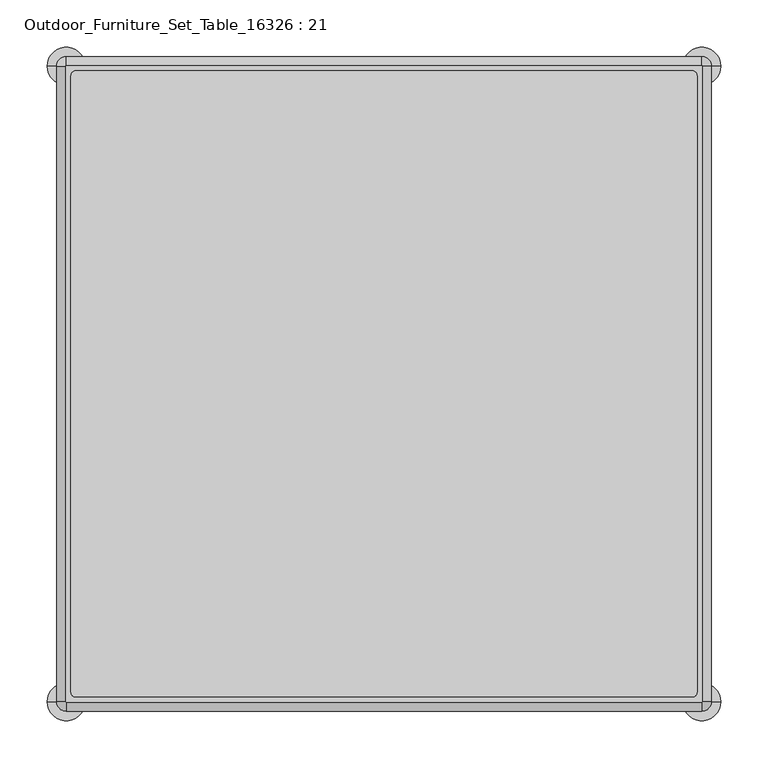
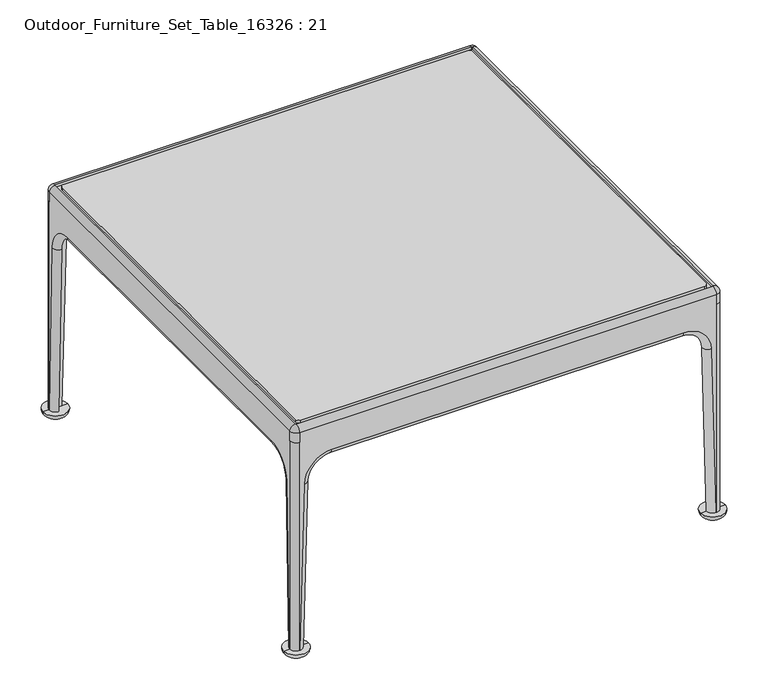
"""IFC4 building model written with IfcOpenShell, lengths in millimetres: furniture geometry, Outdoor_Furniture_Set_Table_16326 : 21."""

from ifc_helpers import new_model, si_unit, point, frame, frame_2d, origin, place, context, project, spatial, polyline, circle_curve, ellipse_curve, trimmed, segment, composite_curve, outline, extrude, source, transform, mapped, element, save
from ifc_brep_helpers import plane_surface, cylinder_surface, revolved_surface, advanced_brep


def outdoor_furniture_set_table_16326_21_ce4fcd7d(model_context):
    return source(origin(), model_context, "Body", "SolidModel", [
        extrude(outline(polyline([(337.0, 337.0), (337.0, -337.0), (-337.0, -337.0), (-337.0, 337.0), (337.0, 337.0)])), frame((0.0, 0.0, 365.0), z_axis=(0.0, 0.0, 1.0), x_axis=(1.0, 0.0, 0.0)), (0.0, 0.0, 1.0), 20.0),
        advanced_brep(
        [(-336.0, 346.0, 10.0), (-326.0034268, 336.0, 9.7382305), (-336.0, 336.0, 10.0), (-328.6370959, 346.0, 291.1779627), (-318.6405227, 336.0, 290.9161932), (-283.6525163, 336.0, 325.0), (283.6525163, 336.0, 325.0), (318.6405227, 336.0, 290.9161932), (326.0034268, 336.0, 9.7382305), (336.0, 336.0, 10.0), (336.0, 336.0, 365.0), (-336.0, 336.0, 365.0), (-283.6525163, 346.0, 335.0), (283.6525163, 346.0, 335.0), (328.6370959, 346.0, 291.1779627), (336.0, 346.0, 10.0), (-336.0, 346.0, 365.0), (-336.0, 346.0, 381.0), (336.0, 346.0, 381.0), (336.0, 346.0, 365.0), (-337.0, -336.0, 365.0), (-336.0, -337.0, 365.0), (336.0, -337.0, 365.0), (337.0, -336.0, 365.0), (337.0, 336.0, 365.0), (336.0, 337.0, 365.0), (-336.0, 337.0, 365.0), (-337.0, 336.0, 365.0), (336.0, -336.0, 365.0), (-336.0, -336.0, 365.0), (-336.0, -346.0, 381.0), (-346.0, -336.0, 381.0), (-346.0, -336.0, 365.0), (-336.0, -346.0, 365.0), (-336.0, -337.0, 390.0), (-337.0, -336.0, 390.0), (-336.0, -346.0, 10.0), (-328.6370853, -346.0, 291.1783664), (-283.6525163, -346.0, 335.0), (283.6525163, -346.0, 335.0), (328.6370853, -346.0, 291.1783664), (336.0, -346.0, 10.0), (336.0, -346.0, 365.0), (336.0, -346.0, 381.0), (336.0, -337.0, 390.0), (346.0, -336.0, 365.0), (346.0, -336.0, 381.0), (337.0, -336.0, 390.0), (346.0, -336.0, 10.0), (346.0, -328.6370959, 291.1779627), (346.0, -283.6525163, 335.0), (346.0, 283.6525163, 335.0), (346.0, 328.6370959, 291.1779627), (346.0, 336.0, 10.0), (346.0, 336.0, 365.0), (346.0, 336.0, 381.0), (337.0, 336.0, 390.0), (336.0, 337.0, 390.0), (-336.0, 337.0, 390.0), (-346.0, 336.0, 365.0), (-346.0, 336.0, 381.0), (-337.0, 336.0, 390.0), (-346.0, 336.0, 10.0), (-346.0, 328.6370853, 291.1783665), (-346.0, 283.6529202, 335.0), (-346.0, -283.6529202, 335.0), (-346.0, -328.6370853, 291.1783665), (-346.0, -336.0, 10.0), (-336.0, -326.0034268, 9.7382305), (-336.0, -336.0, 10.0), (-336.0, -318.6405121, 290.916597), (-336.0, -283.6529202, 325.0), (-336.0, 283.6529202, 325.0), (-336.0, 318.6405121, 290.916597), (-336.0, 326.0034268, 9.7382305), (326.0034268, -336.0, 9.7382305), (336.0, -336.0, 10.0), (318.6405144, -336.0, 290.9165072), (283.6525163, -336.0, 325.0), (-283.6525163, -336.0, 325.0), (-318.6405144, -336.0, 290.9165072), (-326.0034268, -336.0, 9.7382305), (336.0, 326.0034268, 9.7382305), (336.0, 318.6405227, 290.9161932), (336.0, 283.6525163, 325.0), (336.0, -283.6525163, 325.0), (336.0, -318.6405227, 290.9161932), (336.0, -326.0034268, 9.7382305)],
        [
            (0, 1, circle_curve(frame((-336.0, 336.0, 10.0), z_axis=(-0.026176948307757304, 0.0, -0.9996573249755604), x_axis=(0.9996573249755604, 0.0, -0.026176948307757304)), 10.0)),
            (1, 2),
            (2, 0),
            (0, 3),
            (3, 4, circle_curve(frame((-328.6370959, 336.0, 291.1779627), z_axis=(-0.026176948307757304, 0.0, -0.9996573249755604), x_axis=(0.9996573249755604, 0.0, -0.026176948307757304)), 10.0)),
            (4, 1),
            (4, 5, circle_curve(frame((-283.6525163, 336.0, 290.0), z_axis=(0.0, 1.0, 0.0), x_axis=(-0.9996573249749426, 0.0, 0.026176948331344894)), 35.0)),
            (5, 6),
            (6, 7, circle_curve(frame((283.6525163, 336.0, 290.0), z_axis=(0.0, 1.0, 0.0), x_axis=(0.0, 0.0, 1.0)), 35.0)),
            (7, 8),
            (8, 9),
            (9, 10),
            (10, 11),
            (11, 2),
            (3, 12, circle_curve(frame((-283.6525163, 346.0, 290.0), z_axis=(0.0, 1.0, 0.0), x_axis=(-0.9996573249749426, 0.0, 0.026176948331344894)), 45.0)),
            (12, 5, circle_curve(frame((-283.6525163, 336.0, 335.0), z_axis=(-1.0, 0.0, 0.0), x_axis=(0.0, 0.0, -1.0)), 10.0)),
            (12, 13),
            (13, 6, circle_curve(frame((283.6525163, 336.0, 335.0), z_axis=(-1.0, 0.0, 0.0), x_axis=(0.0, 0.0, -1.0)), 10.0)),
            (13, 14, circle_curve(frame((283.6525163, 346.0, 290.0), z_axis=(0.0, 1.0, 0.0), x_axis=(0.0, 0.0, 1.0)), 45.0)),
            (14, 7, circle_curve(frame((328.6370959, 336.0, 291.1779627), z_axis=(-0.02617694833120655, 0.0, 0.9996573249749463), x_axis=(-0.9996573249749463, 0.0, -0.02617694833120655)), 10.0)),
            (8, 15, circle_curve(frame((336.0, 336.0, 10.0), z_axis=(0.026176948307756947, 0.0, -0.9996573249755604), x_axis=(-0.9996573249755604, 0.0, -0.026176948307756947)), 10.0)),
            (15, 9),
            (14, 15),
            (0, 16),
            (16, 17),
            (17, 18),
            (18, 19),
            (19, 15),
            (20, 21, circle_curve(frame((-336.0, -336.0, 365.0), z_axis=(0.0, 0.0, 1.0), x_axis=(-1.0, 0.0, 0.0)), 1.0)),
            (21, 22),
            (22, 23, circle_curve(frame((336.0, -336.0, 365.0), z_axis=(0.0, 0.0, 1.0), x_axis=(0.0, -1.0, 0.0)), 1.0)),
            (23, 24),
            (24, 25, circle_curve(frame((336.0, 336.0, 365.0), z_axis=(0.0, 0.0, 1.0), x_axis=(1.0, 0.0, 0.0)), 1.0)),
            (25, 26),
            (26, 27, circle_curve(frame((-336.0, 336.0, 365.0), z_axis=(0.0, 0.0, 1.0), x_axis=(0.0, 1.0, 0.0)), 1.0)),
            (27, 20),
            (10, 28),
            (28, 29),
            (29, 11),
            (30, 31, circle_curve(frame((-336.0, -336.0, 381.0), z_axis=(0.0, 0.0, -1.0), x_axis=(-1.0, 0.0, 0.0)), 10.0)),
            (31, 32),
            (32, 33, circle_curve(frame((-336.0, -336.0, 365.0), z_axis=(0.0, 0.0, 1.0), x_axis=(-1.0, 0.0, 0.0)), 10.0)),
            (33, 30),
            (30, 34, circle_curve(frame((-336.0, -337.0, 381.0), z_axis=(-1.0, 0.0, 0.0), x_axis=(0.0, 1.0, 0.0)), 9.0)),
            (34, 35, circle_curve(frame((-336.0, -336.0, 390.0), z_axis=(0.0, 0.0, -1.0), x_axis=(-1.0, 0.0, 0.0)), 1.0)),
            (35, 31, circle_curve(frame((-337.0, -336.0, 381.0), z_axis=(0.0, -1.0, 0.0), x_axis=(1.0, 0.0, 0.0)), 9.0)),
            (33, 36),
            (36, 37),
            (37, 38, circle_curve(frame((-283.6525163, -346.0, 290.0), z_axis=(0.0, 1.0, 0.0), x_axis=(0.0, 0.0, 1.0)), 45.0)),
            (38, 39),
            (39, 40, circle_curve(frame((283.6525163, -346.0, 290.0), z_axis=(0.0, 1.0, 0.0), x_axis=(0.9996570900025821, 0.0, 0.026185920025262065)), 45.0)),
            (40, 41),
            (41, 42),
            (42, 43),
            (43, 30),
            (43, 44, circle_curve(frame((336.0, -337.0, 381.0), z_axis=(-1.0, 0.0, 0.0), x_axis=(0.0, 1.0, 0.0)), 9.0)),
            (44, 34),
            (42, 45, circle_curve(frame((336.0, -336.0, 365.0), z_axis=(0.0, 0.0, 1.0), x_axis=(0.0, -1.0, 0.0)), 10.0)),
            (45, 46),
            (46, 43, circle_curve(frame((336.0, -336.0, 381.0), z_axis=(0.0, 0.0, -1.0), x_axis=(0.0, -1.0, 0.0)), 10.0)),
            (46, 47, circle_curve(frame((337.0, -336.0, 381.0), z_axis=(0.0, -1.0, 0.0), x_axis=(-1.0, 0.0, 0.0)), 9.0)),
            (47, 44, circle_curve(frame((336.0, -336.0, 390.0), z_axis=(0.0, 0.0, -1.0), x_axis=(0.0, -1.0, 0.0)), 1.0)),
            (45, 48),
            (48, 49),
            (49, 50, circle_curve(frame((346.0, -283.6525163, 290.0), z_axis=(-1.0, 0.0, 0.0), x_axis=(0.0, 0.0, 1.0)), 45.0)),
            (50, 51),
            (51, 52, circle_curve(frame((346.0, 283.6525163, 290.0), z_axis=(-1.0, 0.0, 0.0), x_axis=(0.0, 0.9996573249749827, 0.0261769483298142)), 45.0)),
            (52, 53),
            (53, 54),
            (54, 55),
            (55, 46),
            (55, 56, circle_curve(frame((337.0, 336.0, 381.0), z_axis=(0.0, -1.0, 0.0), x_axis=(-1.0, 0.0, 0.0)), 9.0)),
            (56, 47),
            (54, 19, circle_curve(frame((336.0, 336.0, 365.0), z_axis=(0.0, 0.0, 1.0), x_axis=(1.0, 0.0, 0.0)), 10.0)),
            (18, 55, circle_curve(frame((336.0, 336.0, 381.0), z_axis=(0.0, 0.0, -1.0), x_axis=(1.0, 0.0, 0.0)), 10.0)),
            (18, 57, circle_curve(frame((336.0, 337.0, 381.0), z_axis=(1.0, 0.0, 0.0), x_axis=(0.0, -1.0, 0.0)), 9.0)),
            (57, 56, circle_curve(frame((336.0, 336.0, 390.0), z_axis=(0.0, 0.0, -1.0), x_axis=(1.0, 0.0, 0.0)), 1.0)),
            (17, 58, circle_curve(frame((-336.0, 337.0, 381.0), z_axis=(1.0, 0.0, 0.0), x_axis=(0.0, -1.0, 0.0)), 9.0)),
            (58, 57),
            (16, 59, circle_curve(frame((-336.0, 336.0, 365.0), z_axis=(0.0, 0.0, 1.0), x_axis=(0.0, 1.0, 0.0)), 10.0)),
            (59, 60),
            (60, 17, circle_curve(frame((-336.0, 336.0, 381.0), z_axis=(0.0, 0.0, -1.0), x_axis=(0.0, 1.0, 0.0)), 10.0)),
            (60, 61, circle_curve(frame((-337.0, 336.0, 381.0), z_axis=(0.0, 1.0, 0.0), x_axis=(1.0, 0.0, 0.0)), 9.0)),
            (61, 58, circle_curve(frame((-336.0, 336.0, 390.0), z_axis=(0.0, 0.0, -1.0), x_axis=(0.0, 1.0, 0.0)), 1.0)),
            (31, 60),
            (59, 62),
            (62, 63),
            (63, 64, circle_curve(frame((-346.0, 283.6529202, 290.0004146), z_axis=(1.0, 0.0, 0.0), x_axis=(0.0, 0.0, 1.0)), 44.9995854)),
            (64, 65),
            (65, 66, circle_curve(frame((-346.0, -283.6529202, 290.0004146), z_axis=(1.0, 0.0, 0.0), x_axis=(0.0, -0.9996573249744442, 0.026176948350383943)), 44.9995854)),
            (66, 67),
            (67, 32),
            (35, 61),
            (34, 21),
            (20, 35),
            (44, 22),
            (47, 23),
            (56, 24),
            (57, 25),
            (58, 26),
            (61, 27),
            (67, 68, circle_curve(frame((-336.0, -336.0, 10.0), z_axis=(0.0, -0.026176948307878527, -0.9996573249755571), x_axis=(0.0, -0.9996573249755571, 0.026176948307878527)), 10.0)),
            (68, 69),
            (69, 67),
            (66, 70, circle_curve(frame((-336.0, -328.6370853, 291.1783665), z_axis=(0.0, -0.026176948307878527, -0.9996573249755571), x_axis=(0.0, -0.9996573249755571, 0.026176948307878527)), 10.0)),
            (70, 68),
            (70, 71, circle_curve(frame((-336.0, -283.6529202, 290.0004146), z_axis=(-1.0, 0.0, 0.0), x_axis=(0.0, -0.9996573249744442, 0.026176948350383943)), 34.9995854)),
            (71, 72),
            (72, 73, circle_curve(frame((-336.0, 283.6529202, 290.0004146), z_axis=(-1.0, 0.0, 0.0), x_axis=(0.0, 0.0, 1.0)), 34.9995854)),
            (73, 74),
            (74, 2),
            (29, 69),
            (65, 71, circle_curve(frame((-336.0, -283.6529202, 335.0), z_axis=(0.0, -1.0, 0.0), x_axis=(0.0, 0.0, 1.0)), 10.0)),
            (64, 72, circle_curve(frame((-336.0, 283.6529202, 335.0), z_axis=(0.0, -1.0, 0.0), x_axis=(0.0, 0.0, 1.0)), 10.0)),
            (63, 73, circle_curve(frame((-336.0, 328.6370853, 291.1783665), z_axis=(0.0, -0.026176948350188068, 0.9996573249744493), x_axis=(0.0, 0.9996573249744493, 0.026176948350188068)), 10.0)),
            (74, 62, circle_curve(frame((-336.0, 336.0, 10.0), z_axis=(0.0, 0.026176948307879942, -0.9996573249755571), x_axis=(0.0, 0.9996573249755571, 0.026176948307879942)), 10.0)),
            (62, 2),
            (41, 75, circle_curve(frame((336.0, -336.0, 10.0), z_axis=(0.026176948314418396, 0.0, -0.999657324975386), x_axis=(-0.999657324975386, 0.0, -0.026176948314418396)), 10.0)),
            (75, 76),
            (76, 41),
            (40, 77, circle_curve(frame((328.6370853, -336.0, 291.1783664), z_axis=(0.02618592002526207, 0.0, -0.9996570900025821), x_axis=(-0.9996570900025821, 0.0, -0.02618592002526207)), 10.0)),
            (77, 75),
            (77, 78, circle_curve(frame((283.6525163, -336.0, 290.0), z_axis=(0.0, -1.0, 0.0), x_axis=(0.9996570900025821, 0.0, 0.026185920025262065)), 35.0)),
            (78, 79),
            (79, 80, circle_curve(frame((-283.6525163, -336.0, 290.0), z_axis=(0.0, -1.0, 0.0), x_axis=(0.0, 0.0, 1.0)), 35.0)),
            (80, 81),
            (81, 69),
            (28, 76),
            (39, 78, circle_curve(frame((283.6525163, -336.0, 335.0), z_axis=(1.0, 0.0, 0.0), x_axis=(0.0, 0.0, -1.0)), 10.0)),
            (38, 79, circle_curve(frame((-283.6525163, -336.0, 335.0), z_axis=(1.0, 0.0, 0.0), x_axis=(0.0, 0.0, -1.0)), 10.0)),
            (37, 80, circle_curve(frame((-328.6370853, -336.0, 291.1783664), z_axis=(0.02618592006476948, 0.0, 0.9996570900015472), x_axis=(0.9996570900015472, 0.0, -0.02618592006476948)), 10.0)),
            (81, 36, circle_curve(frame((-336.0, -336.0, 10.0), z_axis=(-0.02617694831409382, 0.0, -0.9996573249753945), x_axis=(0.9996573249753945, 0.0, -0.02617694831409382)), 10.0)),
            (36, 69),
            (53, 82, circle_curve(frame((336.0, 336.0, 10.0), z_axis=(0.0, 0.026176948307602733, -0.9996573249755644), x_axis=(0.0, -0.9996573249755644, -0.026176948307602733)), 10.0)),
            (82, 9),
            (9, 53),
            (52, 83, circle_curve(frame((336.0, 328.6370959, 291.1779627), z_axis=(0.0, 0.026176948307602733, -0.9996573249755644), x_axis=(0.0, -0.9996573249755644, -0.026176948307602733)), 10.0)),
            (83, 82),
            (83, 84, circle_curve(frame((336.0, 283.6525163, 290.0), z_axis=(1.0, 0.0, 0.0), x_axis=(0.0, 0.9996573249749827, 0.0261769483298142)), 35.0)),
            (84, 85),
            (85, 86, circle_curve(frame((336.0, -283.6525163, 290.0), z_axis=(1.0, 0.0, 0.0), x_axis=(0.0, 0.0, 1.0)), 35.0)),
            (86, 87),
            (87, 76),
            (51, 84, circle_curve(frame((336.0, 283.6525163, 335.0), z_axis=(0.0, 1.0, 0.0), x_axis=(0.0, 0.0, -1.0)), 10.0)),
            (50, 85, circle_curve(frame((336.0, -283.6525163, 335.0), z_axis=(0.0, 1.0, 0.0), x_axis=(0.0, 0.0, -1.0)), 10.0)),
            (49, 86, circle_curve(frame((336.0, -328.6370959, 291.1779627), z_axis=(0.0, 0.026176948331144378, 0.999657324974948), x_axis=(0.0, 0.999657324974948, -0.026176948331144378)), 10.0)),
            (87, 48, circle_curve(frame((336.0, -336.0, 10.0), z_axis=(0.0, -0.0261769483077446, -0.9996573249755608), x_axis=(0.0, 0.9996573249755608, -0.0261769483077446)), 10.0)),
            (48, 76),
            (15, 53, circle_curve(frame((336.0, 336.0, 10.0), z_axis=(0.0, 0.0, -1.0), x_axis=(1.0, 0.0, 0.0)), 10.0)),
            (48, 41, circle_curve(frame((336.0, -336.0, 10.0), z_axis=(0.0, 0.0, -1.0), x_axis=(1.0, 0.0, 0.0)), 10.0)),
            (36, 67, circle_curve(frame((-336.0, -336.0, 10.0), z_axis=(0.0, 0.0, -1.0), x_axis=(1.0, 0.0, 0.0)), 10.0)),
            (62, 0, circle_curve(frame((-336.0, 336.0, 10.0), z_axis=(0.0, 0.0, -1.0), x_axis=(1.0, 0.0, 0.0)), 10.0)),
        ],
        [
            plane_surface(frame((-336.0, 346.0, 10.0), z_axis=(-0.026176948307757304, 0.0, -0.9996573249755604), x_axis=(0.0, 1.0, 0.0))),
            cylinder_surface(frame((-336.0, 336.0, 10.0), z_axis=(-0.026176948307757304, 0.0, -0.9996573249755604), x_axis=(0.9996573249755604, 0.0, -0.026176948307757304)), 10.0),
            plane_surface(frame((-326.0034268, 336.0, 9.7382305), z_axis=(0.0, -1.0, 0.0), x_axis=(0.02617694830775733, 0.0, 0.9996573249755604))),
            revolved_surface(trimmed(ellipse_curve(frame((-328.6370959, 336.0, 291.1779627), z_axis=(-0.026176948331344894, 0.0, -0.9996573249749426), x_axis=(0.9996573249749426, 0.0, -0.026176948331344894)), 10.0, 10.0), [point((-328.6370959, 346.0, 291.1779627))], [point((-318.6405227, 336.0, 290.9161932))], True, "CARTESIAN"), (-283.6525163, 346.0, 290.0), (0.0, 1.0, 0.0)),
            cylinder_surface(frame((-283.6525163, 336.0, 335.0), z_axis=(-1.0, 0.0, 0.0), x_axis=(0.0, 0.0, -1.0)), 10.0),
            revolved_surface(trimmed(ellipse_curve(frame((283.6525163, 336.0, 335.0), z_axis=(-1.0, 0.0, 0.0), x_axis=(0.0, 0.0, -1.0)), 10.0, 10.0), [point((283.6525163, 346.0, 335.0))], [point((283.6525163, 336.0, 325.0))], True, "CARTESIAN"), (283.6525163, 346.0, 290.0), (0.0, 1.0, 0.0)),
            plane_surface(frame((336.0, 346.0, 10.0), z_axis=(0.026176948307756947, 0.0, -0.9996573249755604), x_axis=(0.0, 1.0, 0.0))),
            cylinder_surface(frame((328.6370959, 336.0, 291.1779627), z_axis=(-0.026176948307756947, 0.0, 0.9996573249755604), x_axis=(-0.9996573249755604, 0.0, -0.026176948307756947)), 10.0),
            plane_surface(frame((-283.6525163, 346.0, 335.0), z_axis=(0.0, 1.0, 0.0), x_axis=(-1.0, 0.0, 0.0))),
            plane_surface(frame((-336.0, 346.0, 365.0), z_axis=(0.0, 0.0, 1.0), x_axis=(0.0, -1.0, 0.0))),
            cylinder_surface(frame((-336.0, -336.0, 0.0), z_axis=(0.0, 0.0, 1.0), x_axis=(-1.0, 0.0, 0.0)), 10.0),
            revolved_surface(trimmed(ellipse_curve(frame((-337.0, -336.0, 381.0), z_axis=(0.0, 1.0, 0.0), x_axis=(1.0, 0.0, 0.0)), 9.0, 9.0), [point((-346.0, -336.0, 381.0))], [point((-337.0, -336.0, 390.0))], True, "CARTESIAN"), (-336.0, -336.0, 0.0), (0.0, 0.0, 1.0)),
            plane_surface(frame((-336.0, -346.0, 365.0), z_axis=(0.0, -1.0, 0.0), x_axis=(1.0, 0.0, 0.0))),
            cylinder_surface(frame((-336.0, -337.0, 381.0), z_axis=(-1.0, 0.0, 0.0), x_axis=(0.0, 1.0, 0.0)), 9.0),
            cylinder_surface(frame((336.0, -336.0, 0.0), z_axis=(0.0, 0.0, 1.0), x_axis=(0.0, -1.0, 0.0)), 10.0),
            revolved_surface(trimmed(ellipse_curve(frame((336.0, -337.0, 381.0), z_axis=(-1.0, 0.0, 0.0), x_axis=(0.0, 1.0, 0.0)), 9.0, 9.0), [point((336.0, -346.0, 381.0))], [point((336.0, -337.0, 390.0))], True, "CARTESIAN"), (336.0, -336.0, 0.0), (0.0, 0.0, 1.0)),
            plane_surface(frame((346.0, -336.0, 365.0), z_axis=(1.0, 0.0, 0.0), x_axis=(0.0, 1.0, 0.0))),
            cylinder_surface(frame((337.0, -336.0, 381.0), z_axis=(0.0, -1.0, 0.0), x_axis=(-1.0, 0.0, 0.0)), 9.0),
            cylinder_surface(frame((336.0, 336.0, 0.0), z_axis=(0.0, 0.0, 1.0), x_axis=(1.0, 0.0, 0.0)), 10.0),
            revolved_surface(trimmed(ellipse_curve(frame((337.0, 336.0, 381.0), z_axis=(0.0, -1.0, 0.0), x_axis=(-1.0, 0.0, 0.0)), 9.0, 9.0), [point((346.0, 336.0, 381.0))], [point((337.0, 336.0, 390.0))], True, "CARTESIAN"), (336.0, 336.0, 0.0), (0.0, 0.0, 1.0)),
            cylinder_surface(frame((336.0, 337.0, 381.0), z_axis=(1.0, 0.0, 0.0), x_axis=(0.0, -1.0, 0.0)), 9.0),
            cylinder_surface(frame((-336.0, 336.0, 0.0), z_axis=(0.0, 0.0, 1.0), x_axis=(0.0, 1.0, 0.0)), 10.0),
            revolved_surface(trimmed(ellipse_curve(frame((-336.0, 337.0, 381.0), z_axis=(1.0, 0.0, 0.0), x_axis=(0.0, -1.0, 0.0)), 9.0, 9.0), [point((-336.0, 346.0, 381.0))], [point((-336.0, 337.0, 390.0))], True, "CARTESIAN"), (-336.0, 336.0, 0.0), (0.0, 0.0, 1.0)),
            plane_surface(frame((-346.0, 336.0, 365.0), z_axis=(-1.0, 0.0, 0.0), x_axis=(0.0, -1.0, 0.0))),
            cylinder_surface(frame((-337.0, 336.0, 381.0), z_axis=(0.0, 1.0, 0.0), x_axis=(1.0, 0.0, 0.0)), 9.0),
            revolved_surface(polyline([(-337.0, -336.0, 390.0), (-337.0, -336.0, 365.0)]), (-336.0, -336.0, 0.0), (0.0, 0.0, 1.0)),
            plane_surface(frame((-336.0, -337.0, 390.0), z_axis=(0.0, 1.0, 0.0), x_axis=(1.0, 0.0, 0.0))),
            revolved_surface(polyline([(336.0, -337.0, 390.0), (336.0, -337.0, 365.0)]), (336.0, -336.0, 0.0), (0.0, 0.0, 1.0)),
            plane_surface(frame((337.0, -336.0, 390.0), z_axis=(-1.0, 0.0, 0.0), x_axis=(0.0, 1.0, 0.0))),
            revolved_surface(polyline([(337.0, 336.0, 390.0), (337.0, 336.0, 365.0)]), (336.0, 336.0, 0.0), (0.0, 0.0, 1.0)),
            plane_surface(frame((336.0, 337.0, 390.0), z_axis=(0.0, -1.0, 0.0), x_axis=(-1.0, 0.0, 0.0))),
            revolved_surface(polyline([(-336.0, 337.0, 390.0), (-336.0, 337.0, 365.0)]), (-336.0, 336.0, 0.0), (0.0, 0.0, 1.0)),
            plane_surface(frame((-337.0, 336.0, 390.0), z_axis=(1.0, 0.0, 0.0), x_axis=(0.0, -1.0, 0.0))),
            plane_surface(frame((-346.0, -336.0, 10.0), z_axis=(0.0, -0.026176948307878527, -0.9996573249755571), x_axis=(1.0, 0.0, 0.0))),
            cylinder_surface(frame((-336.0, -336.0, 10.0), z_axis=(0.0, -0.026176948307878527, -0.9996573249755571), x_axis=(0.0, -0.9996573249755571, 0.026176948307878527)), 10.0),
            plane_surface(frame((-336.0, -326.0034268, 9.7382305), z_axis=(1.0, 0.0, 0.0), x_axis=(0.0, 0.026176948307878613, 0.9996573249755571))),
            revolved_surface(trimmed(ellipse_curve(frame((-336.0, -328.6370853, 291.1783665), z_axis=(0.0, -0.026176948350383943, -0.9996573249744442), x_axis=(0.0, -0.9996573249744442, 0.026176948350383943)), 10.0, 10.0), [point((-346.0, -328.6370853, 291.1783665))], [point((-336.0, -318.6405121, 290.916597))], True, "CARTESIAN"), (-346.0, -283.6529202, 290.0004146), (-1.0, 0.0, 0.0)),
            cylinder_surface(frame((-336.0, -283.6529202, 335.0), z_axis=(0.0, -1.0, 0.0), x_axis=(0.0, 0.0, 1.0)), 10.0),
            revolved_surface(trimmed(ellipse_curve(frame((-336.0, 283.6529202, 335.0), z_axis=(0.0, -1.0, 0.0), x_axis=(0.0, 0.0, 1.0)), 10.0, 10.0), [point((-346.0, 283.6529202, 335.0))], [point((-336.0, 283.6529202, 325.0))], True, "CARTESIAN"), (-346.0, 283.6529202, 290.0004146), (-1.0, 0.0, 0.0)),
            plane_surface(frame((-346.0, 336.0, 10.0), z_axis=(0.0, 0.026176948307879942, -0.9996573249755571), x_axis=(1.0, 0.0, 0.0))),
            cylinder_surface(frame((-336.0, 328.6370853, 291.1783665), z_axis=(0.0, -0.026176948307879942, 0.9996573249755571), x_axis=(0.0, 0.9996573249755571, 0.026176948307879942)), 10.0),
            plane_surface(frame((336.0, -346.0, 10.0), z_axis=(0.026176948314418396, 0.0, -0.999657324975386), x_axis=(0.0, -1.0, 0.0))),
            cylinder_surface(frame((336.0, -336.0, 10.0), z_axis=(0.026176948314418396, 0.0, -0.999657324975386), x_axis=(-0.999657324975386, 0.0, -0.026176948314418396)), 10.0),
            plane_surface(frame((326.0034268, -336.0, 9.7382305), z_axis=(0.0, 1.0, 0.0), x_axis=(-0.02617694831441851, 0.0, 0.999657324975386))),
            revolved_surface(trimmed(ellipse_curve(frame((328.6370853, -336.0, 291.1783664), z_axis=(0.02618592002526207, 0.0, -0.9996570900025821), x_axis=(-0.9996570900025821, 0.0, -0.02618592002526207)), 10.0, 10.0), [point((328.6370853, -346.0, 291.1783664))], [point((318.6405144, -336.0, 290.9165072))], True, "CARTESIAN"), (283.6525163, -346.0, 290.0), (0.0, -1.0, 0.0)),
            cylinder_surface(frame((283.6525163, -336.0, 335.0), z_axis=(1.0, 0.0, 0.0), x_axis=(0.0, 0.0, -1.0)), 10.0),
            revolved_surface(trimmed(ellipse_curve(frame((-283.6525163, -336.0, 335.0), z_axis=(1.0, 0.0, 0.0), x_axis=(0.0, 0.0, -1.0)), 10.0, 10.0), [point((-283.6525163, -346.0, 335.0))], [point((-283.6525163, -336.0, 325.0))], True, "CARTESIAN"), (-283.6525163, -346.0, 290.0), (0.0, -1.0, 0.0)),
            plane_surface(frame((-336.0, -346.0, 10.0), z_axis=(-0.026176948314093826, 0.0, -0.9996573249753945), x_axis=(0.0, -1.0, 0.0))),
            cylinder_surface(frame((-328.6370853, -336.0, 291.1783664), z_axis=(0.02617694831409382, 0.0, 0.9996573249753945), x_axis=(0.9996573249753945, 0.0, -0.02617694831409382)), 10.0),
            plane_surface(frame((346.0, 336.0, 10.0), z_axis=(0.0, 0.026176948307602733, -0.9996573249755644), x_axis=(1.0, 0.0, 0.0))),
            cylinder_surface(frame((336.0, 336.0, 10.0), z_axis=(0.0, 0.026176948307602733, -0.9996573249755644), x_axis=(0.0, -0.9996573249755644, -0.026176948307602733)), 10.0),
            plane_surface(frame((336.0, 326.0034268, 9.7382305), z_axis=(-1.0, 0.0, 0.0), x_axis=(0.0, -0.02617694830760276, 0.9996573249755644))),
            revolved_surface(trimmed(ellipse_curve(frame((336.0, 328.6370959, 291.1779627), z_axis=(0.0, 0.0261769483298142, -0.9996573249749827), x_axis=(0.0, -0.9996573249749827, -0.0261769483298142)), 10.0, 10.0), [point((346.0, 328.6370959, 291.1779627))], [point((336.0, 318.6405227, 290.9161932))], True, "CARTESIAN"), (346.0, 283.6525163, 290.0), (1.0, 0.0, 0.0)),
            cylinder_surface(frame((336.0, 283.6525163, 335.0), z_axis=(0.0, 1.0, 0.0), x_axis=(0.0, 0.0, -1.0)), 10.0),
            revolved_surface(trimmed(ellipse_curve(frame((336.0, -283.6525163, 335.0), z_axis=(0.0, 1.0, 0.0), x_axis=(0.0, 0.0, -1.0)), 10.0, 10.0), [point((346.0, -283.6525163, 335.0))], [point((336.0, -283.6525163, 325.0))], True, "CARTESIAN"), (346.0, -283.6525163, 290.0), (1.0, 0.0, 0.0)),
            plane_surface(frame((346.0, -336.0, 10.0), z_axis=(0.0, -0.0261769483077446, -0.9996573249755608), x_axis=(1.0, 0.0, 0.0))),
            cylinder_surface(frame((336.0, -328.6370959, 291.1779627), z_axis=(0.0, 0.0261769483077446, 0.9996573249755608), x_axis=(0.0, 0.9996573249755608, -0.0261769483077446)), 10.0),
            plane_surface(frame((336.0, 336.0, 10.0), z_axis=(0.0, 0.0, -1.0), x_axis=(-1.0, 0.0, 0.0))),
            cylinder_surface(frame((336.0, 336.0, 10.0), z_axis=(0.0, 0.0, 1.0), x_axis=(1.0, 0.0, 0.0)), 10.0),
            cylinder_surface(frame((336.0, -336.0, 0.0), z_axis=(0.0, 0.0, 1.0), x_axis=(1.0, 0.0, 0.0)), 10.0),
            cylinder_surface(frame((-336.0, -336.0, 0.0), z_axis=(0.0, 0.0, 1.0), x_axis=(1.0, 0.0, 0.0)), 10.0),
            cylinder_surface(frame((-336.0, 336.0, 0.0), z_axis=(0.0, 0.0, 1.0), x_axis=(1.0, 0.0, 0.0)), 10.0),
        ],
        [
            (0, [[1, 2, 3]]),
            (1, [[-1, 4, 5, 6]]),
            (2, [[-2, -6, 7, 8, 9, 10, 11, 12, 13, 14]]),
            (3, [[-5, 15, 16, -7]]),
            (4, [[-8, -16, 17, 18]]),
            (5, [[-9, -18, 19, 20]]),
            (6, [[-11, 21, 22]]),
            (7, [[-10, -20, 23, -21]]),
            (8, [[-4, 24, 25, 26, 27, 28, -23, -19, -17, -15]]),
            (9, [[29, 30, 31, 32, 33, 34, 35, 36], [-13, 37, 38, 39]]),
            (10, [[40, 41, 42, 43]]),
            (11, [[-40, 44, 45, 46]]),
            (12, [[-43, 47, 48, 49, 50, 51, 52, 53, 54, 55]]),
            (13, [[-44, -55, 56, 57]]),
            (14, [[-54, 58, 59, 60]]),
            (15, [[-56, -60, 61, 62]]),
            (16, [[-59, 63, 64, 65, 66, 67, 68, 69, 70, 71]]),
            (17, [[-61, -71, 72, 73]]),
            (18, [[-70, 74, -27, 75]]),
            (19, [[-72, -75, 76, 77]]),
            (20, [[-76, -26, 78, 79]]),
            (21, [[-25, 80, 81, 82]]),
            (22, [[-78, -82, 83, 84]]),
            (23, [[-41, 85, -81, 86, 87, 88, 89, 90, 91, 92]]),
            (24, [[-46, 93, -83, -85]]),
            (25, [[-45, 94, -29, 95]]),
            (26, [[-57, 96, -30, -94]]),
            (27, [[-62, 97, -31, -96]]),
            (28, [[-73, 98, -32, -97]]),
            (29, [[-77, 99, -33, -98]]),
            (30, [[-79, 100, -34, -99]]),
            (31, [[-84, 101, -35, -100]]),
            (32, [[-93, -95, -36, -101]]),
            (33, [[102, 103, 104]]),
            (34, [[-102, -91, 105, 106]]),
            (35, [[-103, -106, 107, 108, 109, 110, 111, -14, -39, 112]]),
            (36, [[-105, -90, 113, -107]]),
            (37, [[-108, -113, -89, 114]]),
            (38, [[-109, -114, -88, 115]]),
            (39, [[-111, 116, 117]]),
            (40, [[-110, -115, -87, -116]]),
            (41, [[118, 119, 120]]),
            (42, [[-118, -52, 121, 122]]),
            (43, [[-119, -122, 123, 124, 125, 126, 127, -112, -38, 128]]),
            (44, [[-121, -51, 129, -123]]),
            (45, [[-124, -129, -50, 130]]),
            (46, [[-125, -130, -49, 131]]),
            (47, [[-127, 132, 133]]),
            (48, [[-126, -131, -48, -132]]),
            (49, [[134, 135, 136]]),
            (50, [[-134, -68, 137, 138]]),
            (51, [[-135, -138, 139, 140, 141, 142, 143, -128, -37, -12]]),
            (52, [[-137, -67, 144, -139]]),
            (53, [[-140, -144, -66, 145]]),
            (54, [[-141, -145, -65, 146]]),
            (55, [[-143, 147, 148]]),
            (56, [[-142, -146, -64, -147]]),
            (57, [[149, -136, -22]]),
            (57, [[150, -120, -148]]),
            (57, [[151, -104, -133]]),
            (57, [[152, -3, -117]]),
            (58, [[-149, -28, -74, -69]]),
            (59, [[-150, -63, -58, -53]]),
            (60, [[-151, -47, -42, -92]]),
            (61, [[-152, -86, -80, -24]]),
        ],
    ),
        extrude(outline(composite_curve([segment(polyline([(326.0228318, -331.0), (-326.0, -331.0)]), True, "CONTINUOUS"), segment(trimmed(circle_curve(frame_2d((-326.0, -326.0)), 5.0), [point((-326.0, -331.0))], [point((-331.0, -326.0))], False, "CARTESIAN"), True, "CONTINUOUS"), segment(polyline([(-331.0, -326.0), (-331.0, 326.0)]), True, "CONTINUOUS"), segment(trimmed(circle_curve(frame_2d((-326.0, 326.0)), 5.0), [point((-331.0, 326.0))], [point((-326.0, 331.0))], False, "CARTESIAN"), True, "CONTINUOUS"), segment(polyline([(-326.0, 331.0), (326.0228318, 331.0)]), True, "CONTINUOUS"), segment(trimmed(circle_curve(frame_2d((326.0228318, 326.0)), 5.0), [point((326.0228318, 331.0))], [point((331.0228318, 326.0))], False, "CARTESIAN"), True, "CONTINUOUS"), segment(polyline([(331.0228318, 326.0), (331.0228318, -326.0)]), True, "CONTINUOUS"), segment(trimmed(circle_curve(frame_2d((326.0228318, -326.0)), 5.0), [point((331.0228318, -326.0))], [point((326.0228318, -331.0))], False, "CARTESIAN"), True, "CONTINUOUS")], self_intersect=False)), frame((0.0, 0.0, 385.0), z_axis=(0.0, 0.0, 1.0), x_axis=(1.0, 0.0, 0.0)), (0.0, 0.0, 1.0), 5.0),
        advanced_brep(
        [(-316.0, -336.0, 10.0), (-356.0, -336.0, 10.0), (-336.0, -336.0, 10.0), (-326.0, -336.0, 0.0), (-346.0, -336.0, 0.0), (-336.0, -336.0, 0.0)],
        [
            (0, 1, circle_curve(frame((-336.0, -336.0, 10.0), z_axis=(0.0, 0.0, 1.0), x_axis=(-1.0, 0.0, 0.0)), 20.0)),
            (1, 2),
            (2, 0),
            (1, 0, circle_curve(frame((-336.0, -336.0, 10.0), z_axis=(0.0, 0.0, 1.0), x_axis=(-1.0, 0.0, 0.0)), 20.0)),
            (3, 4, circle_curve(frame((-336.0, -336.0, 0.0), z_axis=(0.0, 0.0, 1.0), x_axis=(-1.0, 0.0, 0.0)), 10.0)),
            (4, 1, circle_curve(frame((-346.0, -336.0, 10.0), z_axis=(0.0, 1.0, 0.0), x_axis=(-1.0, 0.0, 0.0)), 10.0)),
            (0, 3, circle_curve(frame((-326.0, -336.0, 10.0), z_axis=(0.0, 1.0, 0.0), x_axis=(1.0, 0.0, 0.0)), 10.0)),
            (4, 3, circle_curve(frame((-336.0, -336.0, 0.0), z_axis=(0.0, 0.0, 1.0), x_axis=(-1.0, 0.0, 0.0)), 10.0)),
            (5, 4),
            (3, 5),
        ],
        [
            plane_surface(frame((-336.0, -336.0, 10.0), z_axis=(0.0, 0.0, 1.0), x_axis=(-1.0, 0.0, 0.0))),
            revolved_surface(trimmed(ellipse_curve(frame((-346.0, -336.0, 10.0), z_axis=(0.0, -1.0, 0.0), x_axis=(-1.0, 0.0, 0.0)), 10.0, 10.0), [point((-356.0, -336.0, 10.0))], [point((-346.0, -336.0, 0.0))], True, "CARTESIAN"), (-336.0, -336.0, 2438.4), (0.0, 0.0, -1.0)),
            plane_surface(frame((-336.0, -336.0, 0.0), z_axis=(0.0, 0.0, -1.0), x_axis=(-1.0, 0.0, 0.0))),
        ],
        [
            (0, [[1, 2, 3]]),
            (0, [[4, -3, -2]]),
            (1, [[5, 6, -1, 7]]),
            (1, [[8, -7, -4, -6]]),
            (2, [[9, -5, 10]]),
            (2, [[-10, -8, -9]]),
        ],
    ),
        advanced_brep(
        [(326.0, -336.0, 0.0), (346.0, -336.0, 0.0), (336.0, -336.0, 0.0), (316.0, -336.0, 10.0), (356.0, -336.0, 10.0), (336.0, -336.0, 10.0)],
        [
            (0, 1, circle_curve(frame((336.0, -336.0, 0.0), z_axis=(0.0, 0.0, -1.0), x_axis=(1.0, 0.0, 0.0)), 10.0)),
            (1, 2),
            (2, 0),
            (1, 0, circle_curve(frame((336.0, -336.0, 0.0), z_axis=(0.0, 0.0, -1.0), x_axis=(1.0, 0.0, 0.0)), 10.0)),
            (3, 4, circle_curve(frame((336.0, -336.0, 10.0), z_axis=(0.0, 0.0, -1.0), x_axis=(1.0, 0.0, 0.0)), 20.0)),
            (4, 1, circle_curve(frame((346.0, -336.0, 10.0), z_axis=(0.0, 1.0, 0.0), x_axis=(-1.0, 0.0, 0.0)), 10.0)),
            (0, 3, circle_curve(frame((326.0, -336.0, 10.0), z_axis=(0.0, 1.0, 0.0), x_axis=(1.0, 0.0, 0.0)), 10.0)),
            (4, 3, circle_curve(frame((336.0, -336.0, 10.0), z_axis=(0.0, 0.0, -1.0), x_axis=(1.0, 0.0, 0.0)), 20.0)),
            (5, 4),
            (3, 5),
        ],
        [
            plane_surface(frame((336.0, -336.0, 0.0), z_axis=(0.0, 0.0, -1.0), x_axis=(1.0, 0.0, 0.0))),
            revolved_surface(trimmed(ellipse_curve(frame((346.0, -336.0, 10.0), z_axis=(0.0, -1.0, 0.0), x_axis=(-1.0, 0.0, 0.0)), 10.0, 10.0), [point((346.0, -336.0, 0.0))], [point((356.0, -336.0, 10.0))], True, "CARTESIAN"), (336.0, -336.0, 2438.4), (0.0, 0.0, 1.0)),
            plane_surface(frame((336.0, -336.0, 10.0), z_axis=(0.0, 0.0, 1.0), x_axis=(1.0, 0.0, 0.0))),
        ],
        [
            (0, [[1, 2, 3]]),
            (0, [[4, -3, -2]]),
            (1, [[5, 6, -1, 7]]),
            (1, [[8, -7, -4, -6]]),
            (2, [[9, -5, 10]]),
            (2, [[-10, -8, -9]]),
        ],
    ),
        advanced_brep(
        [(316.0, 336.0, 10.0), (356.0, 336.0, 10.0), (336.0, 336.0, 10.0), (326.0, 336.0, 0.0), (346.0, 336.0, 0.0), (336.0, 336.0, 0.0)],
        [
            (0, 1, circle_curve(frame((336.0, 336.0, 10.0), z_axis=(0.0, 0.0, 1.0), x_axis=(1.0, 0.0, 0.0)), 20.0)),
            (1, 2),
            (2, 0),
            (1, 0, circle_curve(frame((336.0, 336.0, 10.0), z_axis=(0.0, 0.0, 1.0), x_axis=(1.0, 0.0, 0.0)), 20.0)),
            (3, 4, circle_curve(frame((336.0, 336.0, 0.0), z_axis=(0.0, 0.0, 1.0), x_axis=(1.0, 0.0, 0.0)), 10.0)),
            (4, 1, circle_curve(frame((346.0, 336.0, 10.0), z_axis=(0.0, -1.0, 0.0), x_axis=(-1.0, 0.0, 0.0)), 10.0)),
            (0, 3, circle_curve(frame((326.0, 336.0, 10.0), z_axis=(0.0, -1.0, 0.0), x_axis=(1.0, 0.0, 0.0)), 10.0)),
            (4, 3, circle_curve(frame((336.0, 336.0, 0.0), z_axis=(0.0, 0.0, 1.0), x_axis=(1.0, 0.0, 0.0)), 10.0)),
            (5, 4),
            (3, 5),
        ],
        [
            plane_surface(frame((336.0, 336.0, 10.0), z_axis=(0.0, 0.0, 1.0), x_axis=(1.0, 0.0, 0.0))),
            revolved_surface(trimmed(ellipse_curve(frame((346.0, 336.0, 10.0), z_axis=(0.0, 1.0, 0.0), x_axis=(-1.0, 0.0, 0.0)), 10.0, 10.0), [point((356.0, 336.0, 10.0))], [point((346.0, 336.0, 0.0))], True, "CARTESIAN"), (336.0, 336.0, 2438.4), (0.0, 0.0, -1.0)),
            plane_surface(frame((336.0, 336.0, 0.0), z_axis=(0.0, 0.0, -1.0), x_axis=(1.0, 0.0, 0.0))),
        ],
        [
            (0, [[1, 2, 3]]),
            (0, [[4, -3, -2]]),
            (1, [[5, 6, -1, 7]]),
            (1, [[8, -7, -4, -6]]),
            (2, [[9, -5, 10]]),
            (2, [[-10, -8, -9]]),
        ],
    ),
        advanced_brep(
        [(-336.0, 336.0, 10.0), (-356.0, 336.0, 10.0), (-316.0, 336.0, 10.0), (-326.0, 336.0, 0.0), (-346.0, 336.0, 0.0), (-336.0, 336.0, 0.0)],
        [
            (0, 1),
            (1, 2, circle_curve(frame((-336.0, 336.0, 10.0), z_axis=(0.0, 0.0, 1.0), x_axis=(-1.0, 0.0, 0.0)), 20.0)),
            (2, 0),
            (2, 1, circle_curve(frame((-336.0, 336.0, 10.0), z_axis=(0.0, 0.0, 1.0), x_axis=(-1.0, 0.0, 0.0)), 20.0)),
            (3, 4, circle_curve(frame((-336.0, 336.0, 0.0), z_axis=(0.0, 0.0, -1.0), x_axis=(-1.0, 0.0, 0.0)), 10.0)),
            (4, 5),
            (5, 3),
            (4, 3, circle_curve(frame((-336.0, 336.0, 0.0), z_axis=(0.0, 0.0, -1.0), x_axis=(-1.0, 0.0, 0.0)), 10.0)),
            (1, 4, circle_curve(frame((-346.0, 336.0, 10.0), z_axis=(0.0, -1.0, 0.0), x_axis=(-1.0, 0.0, 0.0)), 10.0)),
            (3, 2, circle_curve(frame((-326.0, 336.0, 10.0), z_axis=(0.0, -1.0, 0.0), x_axis=(1.0, 0.0, 0.0)), 10.0)),
        ],
        [
            plane_surface(frame((-336.0, 336.0, 10.0), z_axis=(0.0, 0.0, 1.0), x_axis=(-1.0, 0.0, 0.0))),
            plane_surface(frame((-336.0, 336.0, 0.0), z_axis=(0.0, 0.0, -1.0), x_axis=(-1.0, 0.0, 0.0))),
            revolved_surface(trimmed(ellipse_curve(frame((-346.0, 336.0, 10.0), z_axis=(0.0, 1.0, 0.0), x_axis=(-1.0, 0.0, 0.0)), 10.0, 10.0), [point((-346.0, 336.0, 0.0))], [point((-356.0, 336.0, 10.0))], True, "CARTESIAN"), (-336.0, 336.0, 2438.4), (0.0, 0.0, 1.0)),
        ],
        [
            (0, [[1, 2, 3]]),
            (0, [[-3, 4, -1]]),
            (1, [[5, 6, 7]]),
            (1, [[8, -7, -6]]),
            (2, [[-2, 9, -5, 10]]),
            (2, [[-4, -10, -8, -9]]),
        ],
    ),
    ])


if __name__ == "__main__":
    model = new_model("IFC4")
    model_context = context("Model", 3, world=origin())
    ifc_project = project(units=[si_unit("LENGTHUNIT", "METRE", prefix="MILLI")], contexts=[model_context])
    site = spatial("IfcSite", under=ifc_project)
    building = spatial("IfcBuilding", under=site)
    placement = place(None, origin())
    outdoor_furniture_set_table_16326_21_shape = outdoor_furniture_set_table_16326_21_ce4fcd7d(model_context)
    element("IfcFurniture", 1, ObjectType="Outdoor_Furniture_Set_Table_16326 : 21", at=placement, inside=building, context=model_context, shape_type="MappedRepresentation", body=[
        mapped(outdoor_furniture_set_table_16326_21_shape, transform((0.0, 0.0, 0.0), x_axis=(1.0, 0.0, 0.0), y_axis=(0.0, 1.0, 0.0), z_axis=(0.0, 0.0, 1.0))),
    ])
    save(model, "model.ifc")

# Revit data of these elements
# Type "Outdoor_Furniture_Set_Table_16326 : 21"
#   Manufacturer = "Knoll"
#   Description = "1966 by Richard Schultz"
#   Width = 0.692 m
#   O = 0.007363 m
#   Height = 0.39 m
#   Depth = 0.692 m
#   AL = 0.043822 m
#   Frame Material = Furniture - Paint - White Gloss
#   Assembly Code = ""
# Element 1 (IfcFurniture, "Outdoor_Furniture_Set_Table_16326 : 21")
#   Materials on its faces: "Furniture - Paint - White Gloss"
# Materials
#   "Furniture - Paint - White Gloss": class "Paint", colour RGB 255 255 255, transparency 0
